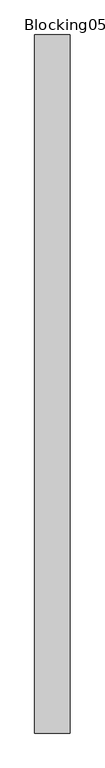
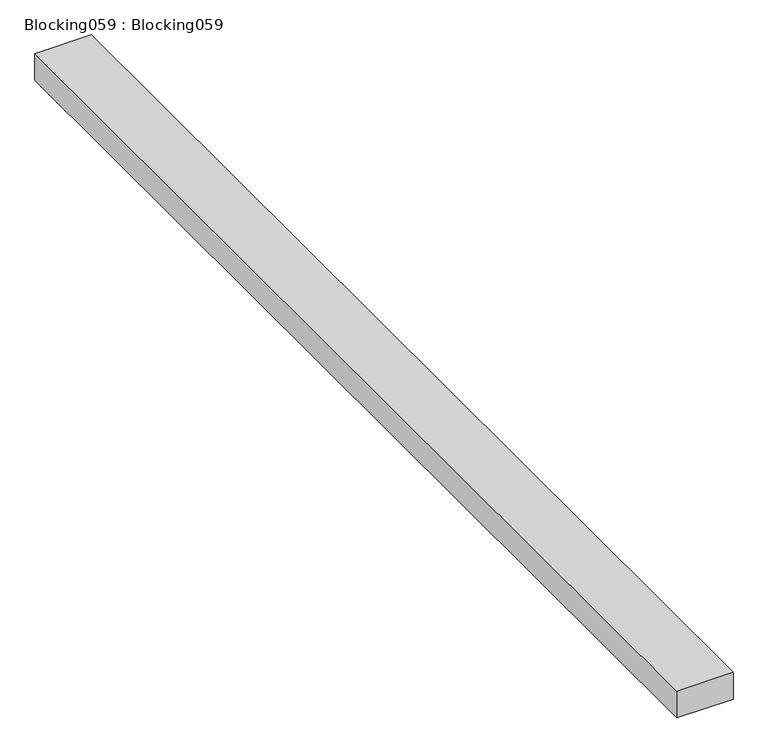
"""IFC4 building model written with IfcOpenShell, lengths in millimetres: proxy geometry, Blocking059 : Blocking059."""

from ifc_helpers import new_model, si_unit, frame, origin, place, context, project, spatial, polyline, outline, extrude, source, transform, mapped, element, save


def blocking059_blocking059_e9c7debe(model_context):
    return source(origin(), model_context, "Body", "SweptSolid", [
        extrude(outline(polyline([(-7121.5276325, 7982.1531721), (-7223.1276325, 7982.1531721), (-7223.1276325, 9982.1531721), (-7121.5276325, 9982.1531721), (-7121.5276325, 7982.1531721)])), frame((0.0, 0.0, 40106.3460083), z_axis=(0.0, 0.0, 1.0), x_axis=(1.0, 0.0, 0.0)), (0.0, 0.0, 1.0), 50.8),
    ])


if __name__ == "__main__":
    model = new_model("IFC4")
    model_context = context("Model", 3, world=origin())
    ifc_project = project(units=[si_unit("LENGTHUNIT", "METRE", prefix="MILLI")], contexts=[model_context])
    site = spatial("IfcSite", under=ifc_project)
    building = spatial("IfcBuilding", under=site)
    placement = place(None, origin())
    blocking059_blocking059_shape = blocking059_blocking059_e9c7debe(model_context)
    element("IfcBuildingElementProxy", 1, Name="Blocking059 : Blocking059", ObjectType="Blocking059 : Blocking059", at=placement, inside=building, context=model_context, shape_type="MappedRepresentation", body=[
        mapped(blocking059_blocking059_shape, transform((0.0, 0.0, 0.0), x_axis=(1.0, 0.0, 0.0), y_axis=(0.0, 1.0, 0.0), z_axis=(0.0, 0.0, 1.0))),
    ])
    save(model, "model.ifc")

# Revit data of these elements
# Type "Blocking059 : Blocking059"
#   NameOverride = "Blocking059"
# Element 1 (IfcBuildingElementProxy, "Blocking059 : Blocking059")
#   Materials on its faces: "WOOD BLOCKING AS REQUIRED"
# Materials
#   "WOOD BLOCKING AS REQUIRED": class "Unassigned", colour RGB 166 124 85, transparency 0, Cost = 0
